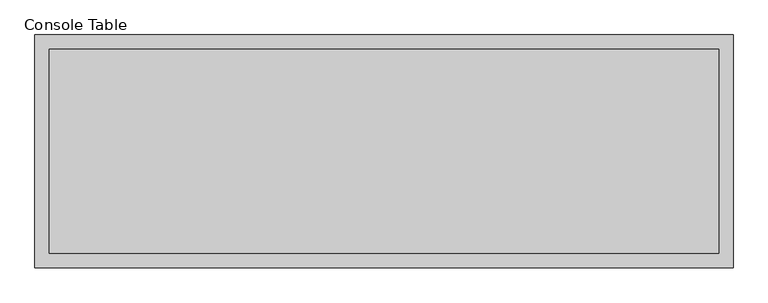
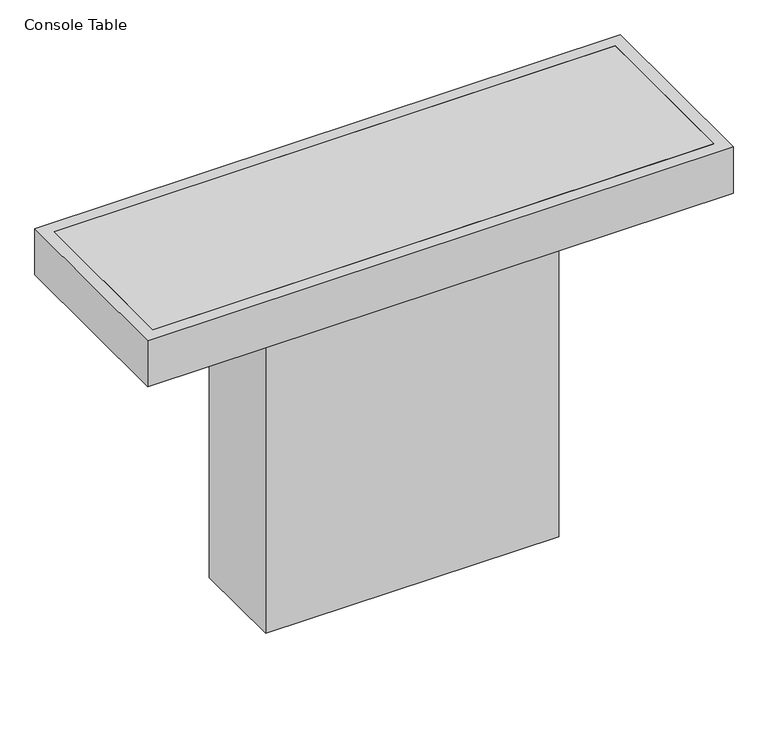
"""IFC4 building model written with IfcOpenShell, lengths in millimetres: furniture geometry, Console Table."""

from ifc_helpers import new_model, si_unit, frame, origin, origin_with_axes, place, context, project, spatial, polyline, outline, extrude, source, transform, mapped, element, save


def console_table_1e0c4b9e(model_context):
    return source(origin(), model_context, "Body", "SweptSolid", [
        extrude(outline(polyline([(304.8, 101.6), (304.8, -101.6), (-304.8, -101.6), (-304.8, 101.6), (304.8, 101.6)])), origin_with_axes(), (0.0, 0.0, 1.0), 787.4),
        extrude(outline(polyline([(-584.2, -177.8), (-584.2, 177.8), (584.2, 177.8), (584.2, -177.8), (-584.2, -177.8)])), frame((0.0, 0.0, 787.4), z_axis=(0.0, 0.0, 1.0), x_axis=(1.0, 0.0, 0.0)), (0.0, 0.0, 1.0), 25.4),
        extrude(outline(polyline([(609.6, 203.2), (609.6, -203.2), (-609.6, -203.2), (-609.6, 203.2), (609.6, 203.2)]), holes=[polyline([(584.2, 177.8), (-584.2, 177.8), (-584.2, -177.8), (584.2, -177.8), (584.2, 177.8)])]), frame((0.0, 0.0, 711.2), z_axis=(0.0, 0.0, 1.0), x_axis=(1.0, 0.0, 0.0)), (0.0, 0.0, 1.0), 101.6),
    ])


if __name__ == "__main__":
    model = new_model("IFC4")
    model_context = context("Model", 3, world=origin())
    ifc_project = project(units=[si_unit("LENGTHUNIT", "METRE", prefix="MILLI")], contexts=[model_context])
    site = spatial("IfcSite", under=ifc_project)
    building = spatial("IfcBuilding", under=site)
    placement = place(None, origin())
    console_table_shape = console_table_1e0c4b9e(model_context)
    element("IfcFurniture", 1, ObjectType="Console Table : 48\" L x 16\" W x 32\" H", at=placement, inside=building, context=model_context, shape_type="MappedRepresentation", body=[
        mapped(console_table_shape, transform((0.0, 0.0, 0.0), x_axis=(1.0, 0.0, 0.0), y_axis=(0.0, 1.0, 0.0), z_axis=(0.0, 0.0, 1.0))),
    ])
    save(model, "model.ifc")

# Revit data of these elements
# Type "Console Table : 48\" L x 16\" W x 32\" H"
#   Table Width = 1' - 4"
#   Table Length = 4' - 0"
#   Table Height = 2' - 8"
#   Pedestal Width = 0' - 8"
#   Pedestal Length = 2' - 0"
#   Frame Thickness = 0' - 1"
#   Frame Height = 0' - 4"
#   Table Surface [instance default] = none
#   Table Frame [instance default] = none
#   Pedestal [instance default] = none
#   Default Elevation = 0
#   Assembly Code = ""
# Element 1 (IfcFurniture, "Console Table : 48\" L x 16\" W x 32\" H")
#   Table Surface = Wood - Teak
#   Table Frame = Steel, Chrome Plated
#   Pedestal = Wood - Teak
#   Materials on its faces: "Wood - Teak", "Steel, Chrome Plated"
# Materials
#   "Wood - Teak": class "Wood", colour RGB 169 114 85, transparency 0, Cost = 0
#   "Steel, Chrome Plated": class "Metal", colour RGB 127 127 127, transparency 0, Description = "Chromiuim plated steel", Cost = 0
